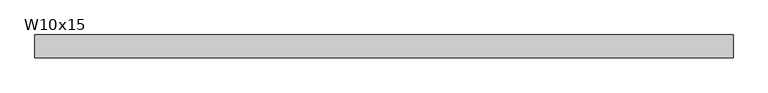
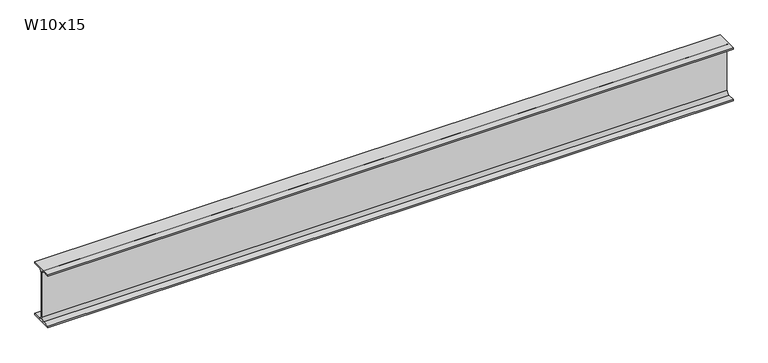
"""IFC4 building model written with IfcOpenShell, lengths in millimetres: beam geometry, RME W-Wide Flange : W10x15."""

from ifc_helpers import new_model, si_unit, point, frame, frame_2d, origin, place, context, project, spatial, polyline, circle_curve, trimmed, segment, composite_curve, outline, extrude, source, transform, mapped, element, save


def w10x15_7efb3c0f(model_context):
    return source(origin(), model_context, "Body", "SweptSolid", [
        extrude(outline(composite_curve([segment(polyline([(50.8, -120.142), (50.8, -127.0), (-50.8, -127.0), (-50.8, -120.142), (-16.7005, -120.142)]), True, "CONTINUOUS"), segment(trimmed(circle_curve(frame_2d((-16.7005, -106.3625)), 13.7795), [point((-16.7005, -120.142))], [point((-2.921, -106.3625))], True, "CARTESIAN"), True, "CONTINUOUS"), segment(polyline([(-2.921, -106.3625), (-2.921, 106.3625)]), True, "CONTINUOUS"), segment(trimmed(circle_curve(frame_2d((-16.7005, 106.3625)), 13.7795), [point((-2.921, 106.3625))], [point((-16.7005, 120.142))], True, "CARTESIAN"), True, "CONTINUOUS"), segment(polyline([(-16.7005, 120.142), (-50.8, 120.142), (-50.8, 127.0), (50.8, 127.0), (50.8, 120.142), (16.7005, 120.142)]), True, "CONTINUOUS"), segment(trimmed(circle_curve(frame_2d((16.7005, 106.3625)), 13.7795), [point((16.7005, 120.142))], [point((2.921, 106.3625))], True, "CARTESIAN"), True, "CONTINUOUS"), segment(polyline([(2.921, 106.3625), (2.921, -106.3625)]), True, "CONTINUOUS"), segment(trimmed(circle_curve(frame_2d((16.7005, -106.3625)), 13.7795), [point((2.921, -106.3625))], [point((16.7005, -120.142))], True, "CARTESIAN"), True, "CONTINUOUS"), segment(polyline([(16.7005, -120.142), (50.8, -120.142)]), True, "CONTINUOUS")], self_intersect=False)), frame((-1594.2534913, 0.0, 0.0), z_axis=(1.0, 0.0, 0.0), x_axis=(0.0, 1.0, 0.0)), (0.0, 0.0, 1.0), 3105.9569826),
    ])


if __name__ == "__main__":
    model = new_model("IFC4")
    model_context = context("Model", 3, world=origin())
    ifc_project = project(units=[si_unit("LENGTHUNIT", "METRE", prefix="MILLI")], contexts=[model_context])
    site = spatial("IfcSite", under=ifc_project)
    building = spatial("IfcBuilding", under=site)
    placement = place(None, origin())
    w10x15_shape = w10x15_7efb3c0f(model_context)
    element("IfcBeam", 1, ObjectType="RME W-Wide Flange : W10x15", at=placement, inside=building, context=model_context, shape_type="MappedRepresentation", body=[
        mapped(w10x15_shape, transform((0.0, 0.0, 0.0), x_axis=(1.0, 0.0, 0.0), y_axis=(0.0, 1.0, 0.0), z_axis=(0.0, 0.0, 1.0))),
    ])
    save(model, "model.ifc")

# Revit data of these elements
# Type "RME W-Wide Flange : W10x15"
#   WELD P [instance default] = ""
#   WELD LE [instance default] = ""
#   WELD D [instance default] = ""
#   TOP SECTION SIZE [instance default] = ""
#   TOP SECTION LENGTH [instance default] = ""
#   REMARKS [instance default] = ""
#   REINF TYPE [instance default] = ""
#   Nominal Size = "W24"
#   End Bearing Capacity [instance default] = ""
#   BOT SECTION SIZE [instance default] = ""
#   BOT SECTION LENGTH [instance default] = ""
#   Assembly Code = "B10"
#   W = 15
#   Start Extension Calculation [instance default] = 10' - 0"
#   Start Extension [instance default] = -0' - 0 1/2"
#   End Extension Calculation [instance default] = 10' - 0"
#   End Extension [instance default] = -0' - 0 1/2"
#   Length [instance default] = 5' - 0"
#   bf = 0' - 4"
#   d = 0' - 10"
#   k = 0' - 0 13/16"
#   k2 = 0' - 0.5425"
#   tf = 0' - 0.27"
#   tw = 0' - 0.23"
#   A = 0.030625 SF
#   Structural Material [instance default] = Metal - Steel - ASTM A992
# Element 1 (IfcBeam, "RME W-Wide Flange : W10x15")
#   Length = 9' - 11.03177"
#   Materials on its faces: "Metal - Steel - ASTM A992"
# Materials
#   "Metal - Steel - ASTM A992": class "Metal", colour RGB 255 128 0, transparency 0
